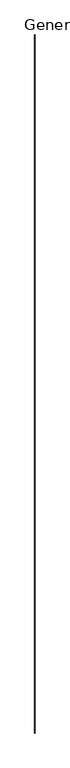
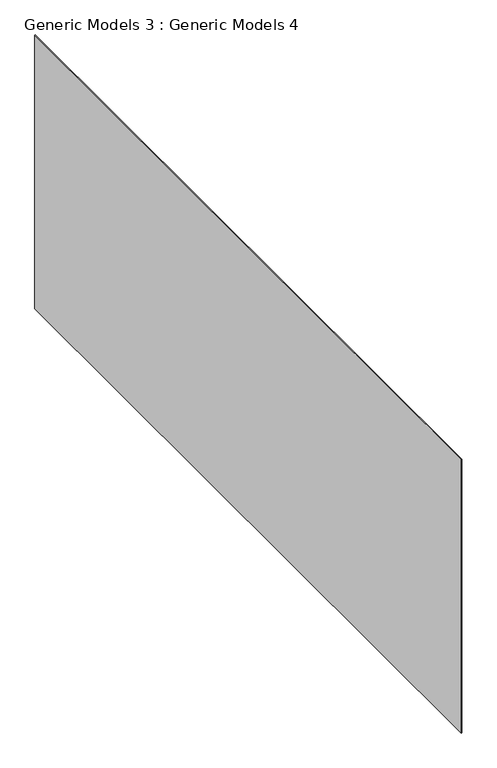
"""IFC4 building model written with IfcOpenShell, lengths in millimetres: proxy geometry, Generic Models 3 : Generic Models 4."""

from ifc_helpers import new_model, si_unit, frame, origin, place, context, project, spatial, polyline, outline, extrude, source, transform, mapped, element, save


def generic_models_3_generic_models_4_3e3b3c38(model_context):
    return source(origin(), model_context, "Body", "SweptSolid", [
        extrude(outline(polyline([(592727.7576893, -527524.3545647), (592727.7576893, -584979.050959), (592702.3576893, -584979.050959), (592702.3576893, -527524.3545647), (592727.7576893, -527524.3545647)])), frame((0.0, 0.0, -2503.337634), z_axis=(0.0, 0.0, 1.0), x_axis=(1.0, 0.0, 0.0)), (0.0, 0.0, 1.0), 22488.6259865),
    ])


if __name__ == "__main__":
    model = new_model("IFC4")
    model_context = context("Model", 3, world=origin())
    ifc_project = project(units=[si_unit("LENGTHUNIT", "METRE", prefix="MILLI")], contexts=[model_context])
    site = spatial("IfcSite", under=ifc_project)
    building = spatial("IfcBuilding", under=site)
    placement = place(None, origin())
    generic_models_3_generic_models_4_shape = generic_models_3_generic_models_4_3e3b3c38(model_context)
    element("IfcBuildingElementProxy", 1, Name="Generic Models 3 : Generic Models 4", ObjectType="Generic Models 3 : Generic Models 4", at=placement, inside=building, context=model_context, shape_type="MappedRepresentation", body=[
        mapped(generic_models_3_generic_models_4_shape, transform((0.0, 0.0, 0.0), x_axis=(1.0, 0.0, 0.0), y_axis=(0.0, 1.0, 0.0), z_axis=(0.0, 0.0, 1.0))),
    ])
    save(model, "model.ifc")

# Revit data of these elements
# Element 1 (IfcBuildingElementProxy, "Generic Models 3 : Generic Models 4")
#   Materials on its faces: "Air"
# Materials
#   "Air": class "Gas", colour RGB 255 255 255, transparency 1, Description = "Air", Cost = 0
